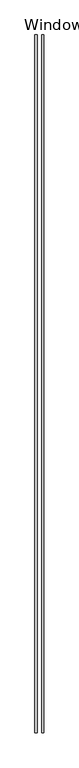
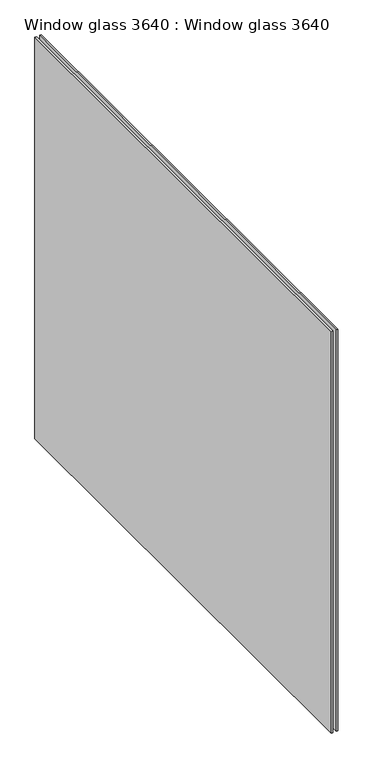
"""IFC4 building model written with IfcOpenShell, lengths in millimetres: proxy geometry, Window glass 3640 : Window glass 3640."""

from ifc_helpers import new_model, si_unit, frame, origin, place, context, project, spatial, polyline, outline, extrude, source, transform, mapped, element, save


def window_glass_3640_window_glass_3640_45d19957(model_context):
    return source(origin(), model_context, "Body", "SweptSolid", [
        extrude(outline(polyline([(-1074.4099125, -1052.890657), (-1080.7345125, -1052.890657), (-1080.7345125, 947.109343), (-1074.4099125, 947.109343), (-1074.4099125, -1052.890657)])), frame((0.0, 0.0, 40362.9028637), z_axis=(0.0, 0.0, 1.0), x_axis=(1.0, 0.0, 0.0)), (0.0, 0.0, 1.0), 1653.9200238),
        extrude(outline(polyline([(-1093.6099125, -1052.890657), (-1099.9345125, -1052.890657), (-1099.9345125, 947.109343), (-1093.6099125, 947.109343), (-1093.6099125, -1052.890657)])), frame((0.0, 0.0, 40362.9028637), z_axis=(0.0, 0.0, 1.0), x_axis=(1.0, 0.0, 0.0)), (0.0, 0.0, 1.0), 1653.9200238),
    ])


if __name__ == "__main__":
    model = new_model("IFC4")
    model_context = context("Model", 3, world=origin())
    ifc_project = project(units=[si_unit("LENGTHUNIT", "METRE", prefix="MILLI")], contexts=[model_context])
    site = spatial("IfcSite", under=ifc_project)
    building = spatial("IfcBuilding", under=site)
    placement = place(None, origin())
    window_glass_3640_window_glass_3640_shape = window_glass_3640_window_glass_3640_45d19957(model_context)
    element("IfcBuildingElementProxy", 1, Name="Window glass 3640 : Window glass 3640", ObjectType="Window glass 3640 : Window glass 3640", at=placement, inside=building, context=model_context, shape_type="MappedRepresentation", body=[
        mapped(window_glass_3640_window_glass_3640_shape, transform((0.0, 0.0, 0.0), x_axis=(1.0, 0.0, 0.0), y_axis=(0.0, 1.0, 0.0), z_axis=(0.0, 0.0, 1.0))),
    ])
    save(model, "model.ifc")

# Revit data of these elements
# Type "Window glass 3640 : Window glass 3640"
#   NameOverride = "Window glass"
# Element 1 (IfcBuildingElementProxy, "Window glass 3640 : Window glass 3640")
#   Materials on its faces: "1\" INSULATED GLAZING"
# Materials
#   "1\" INSULATED GLAZING": class "Unassigned", colour RGB 146 199 212, transparency 0
